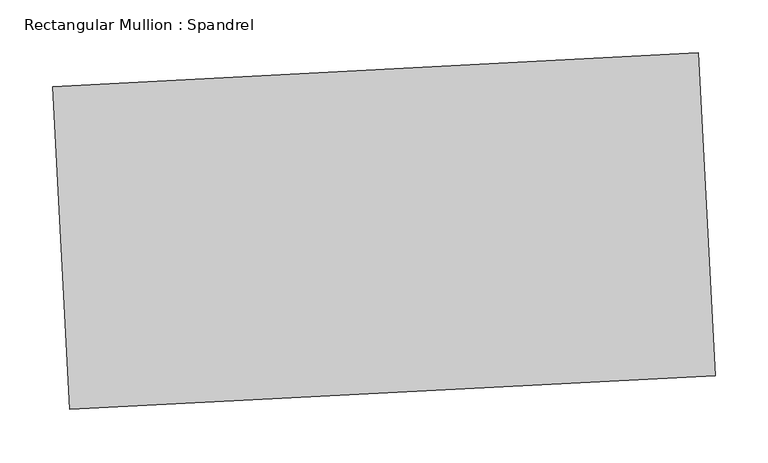
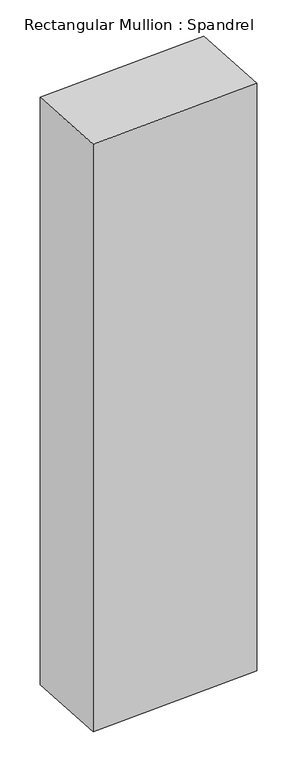
"""IFC4 building model written with IfcOpenShell, lengths in millimetres: member geometry, Rectangular Mullion : Spandrel."""

from ifc_helpers import new_model, si_unit, frame, origin, place, context, project, spatial, polyline, outline, extrude, source, transform, mapped, element, save


def rectangular_mullion_spandrel_dc5cde31(model_context):
    return source(origin(), model_context, "Body", "SweptSolid", [
        extrude(outline(polyline([(-617.1582819, 136.2391416), (-8.3937175, 168.1431406), (7.5582819, -136.2391416), (-601.2062825, -168.1431406), (-617.1582819, 136.2391416)])), frame((0.0, 0.0, -2238.2848233), z_axis=(0.0, 0.0, 1.0), x_axis=(1.0, 0.0, 0.0)), (0.0, 0.0, 1.0), 2238.2848233),
    ])


if __name__ == "__main__":
    model = new_model("IFC4")
    model_context = context("Model", 3, world=origin())
    ifc_project = project(units=[si_unit("LENGTHUNIT", "METRE", prefix="MILLI")], contexts=[model_context])
    site = spatial("IfcSite", under=ifc_project)
    building = spatial("IfcBuilding", under=site)
    placement = place(None, origin())
    rectangular_mullion_spandrel_shape = rectangular_mullion_spandrel_dc5cde31(model_context)
    element("IfcMember", 1, ObjectType="Rectangular Mullion : Spandrel", at=placement, inside=building, context=model_context, shape_type="MappedRepresentation", body=[
        mapped(rectangular_mullion_spandrel_shape, transform((0.0, 0.0, 0.0), x_axis=(1.0, 0.0, 0.0), y_axis=(0.0, 1.0, 0.0), z_axis=(0.0, 0.0, 1.0))),
    ])
    save(model, "model.ifc")

# Revit data of these elements
# Type "Rectangular Mullion : Spandrel"
#   built-in parameter 1007304 = 1 (stored number, unit not read)
#   built-in parameter 1007301 = 1 (stored number, unit not read)
#   built-in parameter 1007300 = 1 (stored number, unit not read)
# Element 1 (IfcMember, "Rectangular Mullion : Spandrel")
#   Materials on its faces: "Aluminum"
# Materials
#   "Aluminum": class "Metal", colour RGB 247 247 247, transparency 0, Description = "Aluminum 6061", Cost = 0
